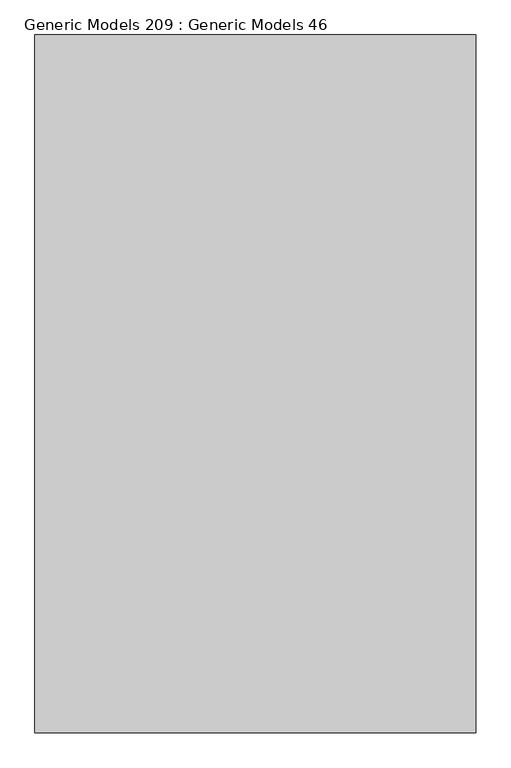
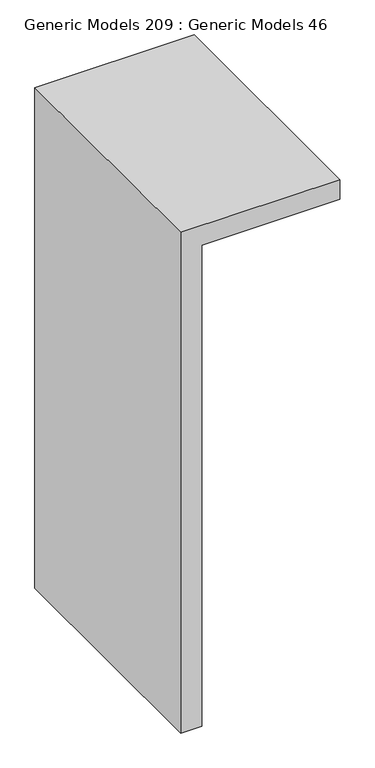
"""IFC4 building model written with IfcOpenShell, lengths in millimetres: proxy geometry, Generic Models 209 : Generic Models 46."""

import ifcopenshell
import ifcopenshell.guid

model = None  # the IFC model being written
_history = None  # IfcOwnerHistory: only IFC2X3 demands one
_inside = {}  # id of a spatial element -> (the spatial element, [elements in it])
_under = {}  # id of a project, library or spatial element -> (it, [spatial elements below it])
_declared = {}  # id of a project -> (the project, [libraries it declares])
_typed = {}  # id of a type object -> (the type object, [elements of that type])
_made_of = {}  # id of a material, layer set ... -> (it, [elements and type objects made of it])


def new_model(schema):
    """Start an empty IFC model of exactly this schema.

    Asked for "IFC4X3", IfcOpenShell would pick the latest addendum, in which some entities
    have other attributes; the version numbers below select the first issue.
    IFC2X3 requires an IfcOwnerHistory on every rooted entity: one is made here for all.
    """
    global model, _history
    if schema == "IFC4X3":
        model = ifcopenshell.file(schema_version=(4, 3, 0, 0))
    else:
        model = ifcopenshell.file(schema=schema)
    _inside.clear()
    _under.clear()
    _declared.clear()
    _typed.clear()
    _made_of.clear()
    _history = None
    if model.schema == "IFC2X3":
        org = make("IfcOrganization", Name="unknown")
        user = make(
            "IfcPersonAndOrganization",
            ThePerson=make("IfcPerson", FamilyName="unknown"),
            TheOrganization=org,
        )
        app = make(
            "IfcApplication",
            ApplicationDeveloper=org,
            Version="unknown",
            ApplicationFullName="unknown",
            ApplicationIdentifier="unknown",
        )
        _history = make(
            "IfcOwnerHistory",
            OwningUser=user,
            OwningApplication=app,
            ChangeAction="ADDED",
            CreationDate=0,
        )
    return model


def make(cls, **values):
    """One entity of the class cls with the attributes given. An attribute that is None is left unset."""
    return model.create_entity(
        cls, **{name: value for name, value in values.items() if value is not None}
    )


def rooted(cls, **values):
    """An entity with a GlobalId (a new one), such as an element, a storey or a relation."""
    return make(cls, GlobalId=ifcopenshell.guid.new(), OwnerHistory=_history, **values)


def si_unit(unit_type, name, prefix=None):
    """IfcSIUnit, for example si_unit("LENGTHUNIT", "METRE", prefix="MILLI")."""
    return make("IfcSIUnit", UnitType=unit_type, Prefix=prefix, Name=name)


def assignment(units):
    """IfcUnitAssignment: the units of a project."""
    return None if units is None else make("IfcUnitAssignment", Units=units)


def point(xyz):
    """IfcCartesianPoint."""
    return None if xyz is None else make("IfcCartesianPoint", Coordinates=xyz)


def direction(xyz):
    """IfcDirection."""
    return None if xyz is None else make("IfcDirection", DirectionRatios=xyz)


def frame(location, z_axis=None, x_axis=None):
    """IfcAxis2Placement3D, a coordinate frame: its origin and axes. An axis left out is left unset."""
    return make(
        "IfcAxis2Placement3D",
        Location=point(location),
        Axis=direction(z_axis),
        RefDirection=direction(x_axis),
    )


def origin():
    """The frame at (0, 0, 0) with its axes left unset."""
    return frame((0.0, 0.0, 0.0))


def place(relative_to, where):
    """IfcLocalPlacement: puts the frame where relative to a parent placement (None: the world)."""
    return make(
        "IfcLocalPlacement", PlacementRelTo=relative_to, RelativePlacement=where
    )


def context(
    kind, dimensions, precision=None, world=None, true_north=None, identifier=None
):
    """IfcGeometricRepresentationContext, for example the 3D "Model" context."""
    return make(
        "IfcGeometricRepresentationContext",
        ContextIdentifier=identifier,
        ContextType=kind,
        CoordinateSpaceDimension=dimensions,
        Precision=precision,
        WorldCoordinateSystem=world,
        TrueNorth=true_north,
    )


def project(units=None, contexts=None):
    """IfcProject with its units and contexts."""
    return rooted(
        "IfcProject",
        Name="project",
        RepresentationContexts=contexts,
        UnitsInContext=assignment(units),
    )


def spatial(cls, under=None, at=None, **own):
    """A site, building, storey or space (cls), placed at a placement, below another one or the project."""
    s = rooted(cls, ObjectPlacement=at, **own)
    if under is not None:
        _under.setdefault(under.id(), (under, []))[1].append(s)
    return s


def polyline(points):
    """IfcPolyline through the points."""
    return make("IfcPolyline", Points=[point(p) for p in points])


def outline(outer, holes=None, kind="AREA"):
    """IfcArbitraryClosedProfileDef: a profile drawn as a closed curve; with holes, ...WithVoids."""
    if holes is None:
        return make("IfcArbitraryClosedProfileDef", ProfileType=kind, OuterCurve=outer)
    return make(
        "IfcArbitraryProfileDefWithVoids",
        ProfileType=kind,
        OuterCurve=outer,
        InnerCurves=holes,
    )


def extrude(swept, where, along, depth):
    """IfcExtrudedAreaSolid: the profile swept, set in the frame where, extruded along a direction by depth."""
    return make(
        "IfcExtrudedAreaSolid",
        SweptArea=swept,
        Position=where,
        ExtrudedDirection=direction(along),
        Depth=depth,
    )


def shape(context_of_items, identifier, shape_type, items):
    """IfcShapeRepresentation: the items that make up one representation, for example the "Body"."""
    return make(
        "IfcShapeRepresentation",
        ContextOfItems=context_of_items,
        RepresentationIdentifier=identifier,
        RepresentationType=shape_type,
        Items=items,
    )


def source(mapping_origin, context_of_items, identifier, shape_type, items):
    """IfcRepresentationMap: a shape defined once, which mapped items show again and again."""
    return make(
        "IfcRepresentationMap",
        MappingOrigin=mapping_origin,
        MappedRepresentation=shape(context_of_items, identifier, shape_type, items),
    )


def transform(
    local_origin,
    x_axis=None,
    y_axis=None,
    z_axis=None,
    scale=None,
    scale2=None,
    scale3=None,
    uniform=True,
):
    """IfcCartesianTransformationOperator3D, or its non-uniform kind. x_axis, y_axis, z_axis: its Axis1, 2, 3."""
    if uniform:
        return make(
            "IfcCartesianTransformationOperator3D",
            Axis1=direction(x_axis),
            Axis2=direction(y_axis),
            LocalOrigin=point(local_origin),
            Scale=scale,
            Axis3=direction(z_axis),
        )
    return make(
        "IfcCartesianTransformationOperator3DnonUniform",
        Axis1=direction(x_axis),
        Axis2=direction(y_axis),
        LocalOrigin=point(local_origin),
        Scale=scale,
        Axis3=direction(z_axis),
        Scale2=scale2,
        Scale3=scale3,
    )


def mapped(mapping_source, mapping_target):
    """IfcMappedItem: shows the shape of a source again, moved by a transform."""
    return make(
        "IfcMappedItem", MappingSource=mapping_source, MappingTarget=mapping_target
    )


def made_of(thing, what):
    """Note that an element or type object is made of a material, layer set ...; save() writes the relation."""
    if what is not None:
        _made_of.setdefault(what.id(), (what, []))[1].append(thing)
    return thing


def element(
    cls,
    number,
    at=None,
    inside=None,
    cuts=None,
    type_object=None,
    material=None,
    context=None,
    identifier="Body",
    shape_type=None,
    held_by="IfcProductDefinitionShape",
    body=None,
    shapes=None,
    **own,
):
    """One element of the class cls, such as IfcWall. Its Tag is "e" and its number.

    at: its placement. inside: the storey or other place that contains it. cuts: it is an
    opening in that element (IfcRelVoidsElement). A single representation is given by context,
    identifier, shape_type and body (its items); several are given by shapes. held_by: the class
    of the entity that holds the representations. save() writes the other relations.
    """
    e = rooted(cls, Tag="e%d" % number, ObjectPlacement=at, **own)
    if body is not None:
        shapes = [shape(context, identifier, shape_type, body)]
    if shapes is not None:
        e.Representation = make(held_by, Representations=shapes)
    if inside is not None:
        _inside.setdefault(inside.id(), (inside, []))[1].append(e)
    if cuts is not None:
        rooted(
            "IfcRelVoidsElement", RelatingBuildingElement=cuts, RelatedOpeningElement=e
        )
    if type_object is not None:
        _typed.setdefault(type_object.id(), (type_object, []))[1].append(e)
    return made_of(e, material)


def aggregate(whole, parts):
    """IfcRelAggregates: a whole, such as a stair, and the parts it consists of."""
    return rooted("IfcRelAggregates", RelatingObject=whole, RelatedObjects=parts)


def save(model, path):
    """Write the relations noted so far, then the file.

    IfcRelAggregates (storeys below a building ...), IfcRelContainedInSpatialStructure (elements
    in a storey), IfcRelDefinesByType, IfcRelAssociatesMaterial and IfcRelDeclares: one each for
    every whole, place, type object, material and project.
    """
    for whole, parts in _under.values():
        aggregate(whole, parts)
    for where, things in _inside.values():
        rooted(
            "IfcRelContainedInSpatialStructure",
            RelatedElements=things,
            RelatingStructure=where,
        )
    for kind, things in _typed.values():
        rooted("IfcRelDefinesByType", RelatedObjects=things, RelatingType=kind)
    for what, things in _made_of.values():
        rooted("IfcRelAssociatesMaterial", RelatedObjects=things, RelatingMaterial=what)
    for by, libraries in _declared.values():
        rooted("IfcRelDeclares", RelatingContext=by, RelatedDefinitions=libraries)
    model.write(path)


def generic_models_209_generic_models_46_b9e04646(model_context):
    return source(origin(), model_context, "Body", "SweptSolid", [
        extrude(outline(polyline([(2559.05, 46689.9625), (2559.05, 45920.025), (0.0, 45920.025), (0.0, 46021.625), (2457.45, 46021.625), (2457.45, 46689.9625), (2559.05, 46689.9625)])), frame((0.0, 0.0, 0.0), z_axis=(0.0, 1.0, 0.0), x_axis=(0.0, 0.0, 1.0)), (0.0, 0.0, 1.0), 1219.2),
    ])


if __name__ == "__main__":
    model = new_model("IFC4")
    model_context = context("Model", 3, world=origin())
    ifc_project = project(units=[si_unit("LENGTHUNIT", "METRE", prefix="MILLI")], contexts=[model_context])
    site = spatial("IfcSite", under=ifc_project)
    building = spatial("IfcBuilding", under=site)
    placement = place(None, origin())
    generic_models_209_generic_models_46_shape = generic_models_209_generic_models_46_b9e04646(model_context)
    element("IfcBuildingElementProxy", 1, Name="Generic Models 209 : Generic Models 46", ObjectType="Generic Models 209 : Generic Models 46", at=placement, inside=building, context=model_context, shape_type="MappedRepresentation", body=[
        mapped(generic_models_209_generic_models_46_shape, transform((0.0, 0.0, 0.0), x_axis=(1.0, 0.0, 0.0), y_axis=(0.0, 1.0, 0.0), z_axis=(0.0, 0.0, 1.0))),
    ])
    save(model, "model.ifc")

# Revit data of these elements
# Element 1 (IfcBuildingElementProxy, "Generic Models 209 : Generic Models 46")
#   Materials on its faces: "EXISTING STRUCTURE"
# Materials
#   "EXISTING STRUCTURE": class "Concrete", colour RGB 129 132 118, transparency 0, Description = "Lightweight concrete", Cost = 0
